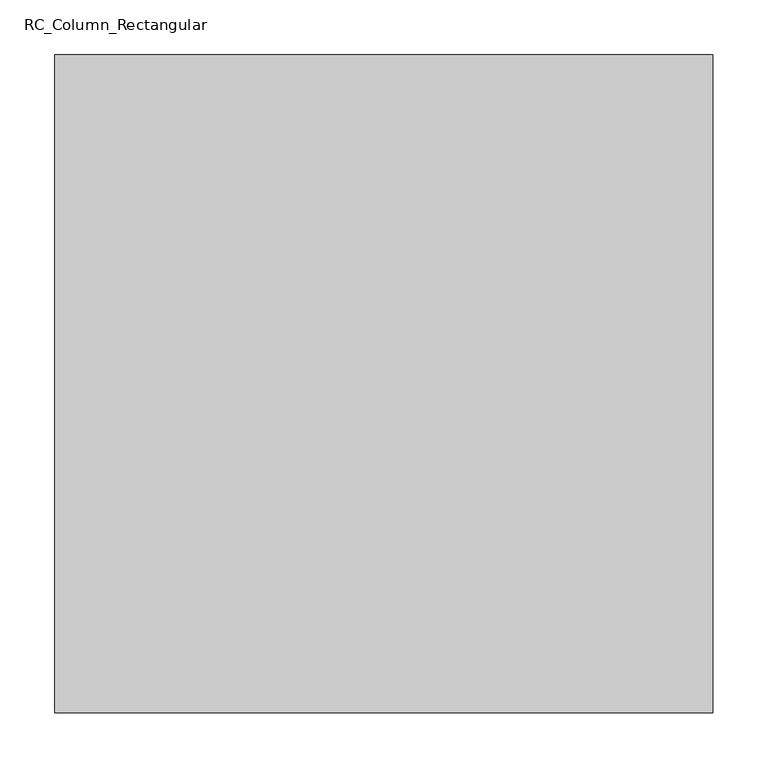
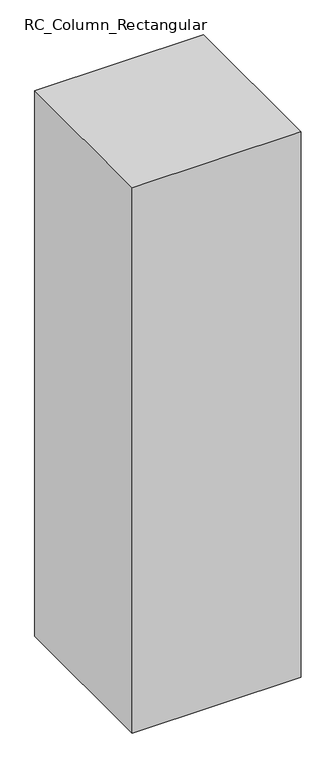
"""IFC4 building model written with IfcOpenShell, lengths in millimetres: column geometry, RC_Column_Rectangular : H_SC_AR_S15_UG PED_W600xL600_Bit_PD2."""

import ifcopenshell
import ifcopenshell.guid

model = None  # the IFC model being written
_history = None  # IfcOwnerHistory: only IFC2X3 demands one
_inside = {}  # id of a spatial element -> (the spatial element, [elements in it])
_under = {}  # id of a project, library or spatial element -> (it, [spatial elements below it])
_declared = {}  # id of a project -> (the project, [libraries it declares])
_typed = {}  # id of a type object -> (the type object, [elements of that type])
_made_of = {}  # id of a material, layer set ... -> (it, [elements and type objects made of it])


def new_model(schema):
    """Start an empty IFC model of exactly this schema.

    Asked for "IFC4X3", IfcOpenShell would pick the latest addendum, in which some entities
    have other attributes; the version numbers below select the first issue.
    IFC2X3 requires an IfcOwnerHistory on every rooted entity: one is made here for all.
    """
    global model, _history
    if schema == "IFC4X3":
        model = ifcopenshell.file(schema_version=(4, 3, 0, 0))
    else:
        model = ifcopenshell.file(schema=schema)
    _inside.clear()
    _under.clear()
    _declared.clear()
    _typed.clear()
    _made_of.clear()
    _history = None
    if model.schema == "IFC2X3":
        org = make("IfcOrganization", Name="unknown")
        user = make(
            "IfcPersonAndOrganization",
            ThePerson=make("IfcPerson", FamilyName="unknown"),
            TheOrganization=org,
        )
        app = make(
            "IfcApplication",
            ApplicationDeveloper=org,
            Version="unknown",
            ApplicationFullName="unknown",
            ApplicationIdentifier="unknown",
        )
        _history = make(
            "IfcOwnerHistory",
            OwningUser=user,
            OwningApplication=app,
            ChangeAction="ADDED",
            CreationDate=0,
        )
    return model


def make(cls, **values):
    """One entity of the class cls with the attributes given. An attribute that is None is left unset."""
    return model.create_entity(
        cls, **{name: value for name, value in values.items() if value is not None}
    )


def rooted(cls, **values):
    """An entity with a GlobalId (a new one), such as an element, a storey or a relation."""
    return make(cls, GlobalId=ifcopenshell.guid.new(), OwnerHistory=_history, **values)


def si_unit(unit_type, name, prefix=None):
    """IfcSIUnit, for example si_unit("LENGTHUNIT", "METRE", prefix="MILLI")."""
    return make("IfcSIUnit", UnitType=unit_type, Prefix=prefix, Name=name)


def assignment(units):
    """IfcUnitAssignment: the units of a project."""
    return None if units is None else make("IfcUnitAssignment", Units=units)


def point(xyz):
    """IfcCartesianPoint."""
    return None if xyz is None else make("IfcCartesianPoint", Coordinates=xyz)


def direction(xyz):
    """IfcDirection."""
    return None if xyz is None else make("IfcDirection", DirectionRatios=xyz)


def frame(location, z_axis=None, x_axis=None):
    """IfcAxis2Placement3D, a coordinate frame: its origin and axes. An axis left out is left unset."""
    return make(
        "IfcAxis2Placement3D",
        Location=point(location),
        Axis=direction(z_axis),
        RefDirection=direction(x_axis),
    )


def origin():
    """The frame at (0, 0, 0) with its axes left unset."""
    return frame((0.0, 0.0, 0.0))


def place(relative_to, where):
    """IfcLocalPlacement: puts the frame where relative to a parent placement (None: the world)."""
    return make(
        "IfcLocalPlacement", PlacementRelTo=relative_to, RelativePlacement=where
    )


def context(
    kind, dimensions, precision=None, world=None, true_north=None, identifier=None
):
    """IfcGeometricRepresentationContext, for example the 3D "Model" context."""
    return make(
        "IfcGeometricRepresentationContext",
        ContextIdentifier=identifier,
        ContextType=kind,
        CoordinateSpaceDimension=dimensions,
        Precision=precision,
        WorldCoordinateSystem=world,
        TrueNorth=true_north,
    )


def project(units=None, contexts=None):
    """IfcProject with its units and contexts."""
    return rooted(
        "IfcProject",
        Name="project",
        RepresentationContexts=contexts,
        UnitsInContext=assignment(units),
    )


def spatial(cls, under=None, at=None, **own):
    """A site, building, storey or space (cls), placed at a placement, below another one or the project."""
    s = rooted(cls, ObjectPlacement=at, **own)
    if under is not None:
        _under.setdefault(under.id(), (under, []))[1].append(s)
    return s


def polyline(points):
    """IfcPolyline through the points."""
    return make("IfcPolyline", Points=[point(p) for p in points])


def outline(outer, holes=None, kind="AREA"):
    """IfcArbitraryClosedProfileDef: a profile drawn as a closed curve; with holes, ...WithVoids."""
    if holes is None:
        return make("IfcArbitraryClosedProfileDef", ProfileType=kind, OuterCurve=outer)
    return make(
        "IfcArbitraryProfileDefWithVoids",
        ProfileType=kind,
        OuterCurve=outer,
        InnerCurves=holes,
    )


def extrude(swept, where, along, depth):
    """IfcExtrudedAreaSolid: the profile swept, set in the frame where, extruded along a direction by depth."""
    return make(
        "IfcExtrudedAreaSolid",
        SweptArea=swept,
        Position=where,
        ExtrudedDirection=direction(along),
        Depth=depth,
    )


def shape(context_of_items, identifier, shape_type, items):
    """IfcShapeRepresentation: the items that make up one representation, for example the "Body"."""
    return make(
        "IfcShapeRepresentation",
        ContextOfItems=context_of_items,
        RepresentationIdentifier=identifier,
        RepresentationType=shape_type,
        Items=items,
    )


def source(mapping_origin, context_of_items, identifier, shape_type, items):
    """IfcRepresentationMap: a shape defined once, which mapped items show again and again."""
    return make(
        "IfcRepresentationMap",
        MappingOrigin=mapping_origin,
        MappedRepresentation=shape(context_of_items, identifier, shape_type, items),
    )


def transform(
    local_origin,
    x_axis=None,
    y_axis=None,
    z_axis=None,
    scale=None,
    scale2=None,
    scale3=None,
    uniform=True,
):
    """IfcCartesianTransformationOperator3D, or its non-uniform kind. x_axis, y_axis, z_axis: its Axis1, 2, 3."""
    if uniform:
        return make(
            "IfcCartesianTransformationOperator3D",
            Axis1=direction(x_axis),
            Axis2=direction(y_axis),
            LocalOrigin=point(local_origin),
            Scale=scale,
            Axis3=direction(z_axis),
        )
    return make(
        "IfcCartesianTransformationOperator3DnonUniform",
        Axis1=direction(x_axis),
        Axis2=direction(y_axis),
        LocalOrigin=point(local_origin),
        Scale=scale,
        Axis3=direction(z_axis),
        Scale2=scale2,
        Scale3=scale3,
    )


def mapped(mapping_source, mapping_target):
    """IfcMappedItem: shows the shape of a source again, moved by a transform."""
    return make(
        "IfcMappedItem", MappingSource=mapping_source, MappingTarget=mapping_target
    )


def made_of(thing, what):
    """Note that an element or type object is made of a material, layer set ...; save() writes the relation."""
    if what is not None:
        _made_of.setdefault(what.id(), (what, []))[1].append(thing)
    return thing


def element(
    cls,
    number,
    at=None,
    inside=None,
    cuts=None,
    type_object=None,
    material=None,
    context=None,
    identifier="Body",
    shape_type=None,
    held_by="IfcProductDefinitionShape",
    body=None,
    shapes=None,
    **own,
):
    """One element of the class cls, such as IfcWall. Its Tag is "e" and its number.

    at: its placement. inside: the storey or other place that contains it. cuts: it is an
    opening in that element (IfcRelVoidsElement). A single representation is given by context,
    identifier, shape_type and body (its items); several are given by shapes. held_by: the class
    of the entity that holds the representations. save() writes the other relations.
    """
    e = rooted(cls, Tag="e%d" % number, ObjectPlacement=at, **own)
    if body is not None:
        shapes = [shape(context, identifier, shape_type, body)]
    if shapes is not None:
        e.Representation = make(held_by, Representations=shapes)
    if inside is not None:
        _inside.setdefault(inside.id(), (inside, []))[1].append(e)
    if cuts is not None:
        rooted(
            "IfcRelVoidsElement", RelatingBuildingElement=cuts, RelatedOpeningElement=e
        )
    if type_object is not None:
        _typed.setdefault(type_object.id(), (type_object, []))[1].append(e)
    return made_of(e, material)


def aggregate(whole, parts):
    """IfcRelAggregates: a whole, such as a stair, and the parts it consists of."""
    return rooted("IfcRelAggregates", RelatingObject=whole, RelatedObjects=parts)


def save(model, path):
    """Write the relations noted so far, then the file.

    IfcRelAggregates (storeys below a building ...), IfcRelContainedInSpatialStructure (elements
    in a storey), IfcRelDefinesByType, IfcRelAssociatesMaterial and IfcRelDeclares: one each for
    every whole, place, type object, material and project.
    """
    for whole, parts in _under.values():
        aggregate(whole, parts)
    for where, things in _inside.values():
        rooted(
            "IfcRelContainedInSpatialStructure",
            RelatedElements=things,
            RelatingStructure=where,
        )
    for kind, things in _typed.values():
        rooted("IfcRelDefinesByType", RelatedObjects=things, RelatingType=kind)
    for what, things in _made_of.values():
        rooted("IfcRelAssociatesMaterial", RelatedObjects=things, RelatingMaterial=what)
    for by, libraries in _declared.values():
        rooted("IfcRelDeclares", RelatingContext=by, RelatedDefinitions=libraries)
    model.write(path)


def rc_column_rectangular_fa199b6f(model_context):
    return source(origin(), model_context, "Body", "SweptSolid", [
        extrude(outline(polyline([(300.0, 300.0), (300.0, -300.0), (-300.0, -300.0), (-300.0, 300.0), (300.0, 300.0)])), frame((0.0, 0.0, -9380.1756499), z_axis=(0.0, 0.0, 1.0), x_axis=(1.0, 0.0, 0.0)), (0.0, 0.0, 1.0), 2050.0),
    ])


if __name__ == "__main__":
    model = new_model("IFC4")
    model_context = context("Model", 3, world=origin())
    ifc_project = project(units=[si_unit("LENGTHUNIT", "METRE", prefix="MILLI")], contexts=[model_context])
    site = spatial("IfcSite", under=ifc_project)
    building = spatial("IfcBuilding", under=site)
    placement = place(None, origin())
    rc_column_rectangular_shape = rc_column_rectangular_fa199b6f(model_context)
    element("IfcColumn", 1, ObjectType="RC_Column_Rectangular : H_SC_AR_S15_UG PED_W600xL600_Bit_PD2", at=placement, inside=building, context=model_context, shape_type="MappedRepresentation", body=[
        mapped(rc_column_rectangular_shape, transform((0.0, 0.0, 0.0), x_axis=(1.0, 0.0, 0.0), y_axis=(0.0, 1.0, 0.0), z_axis=(0.0, 0.0, 1.0))),
    ])
    save(model, "model.ifc")

# Revit data of these elements
# Type "RC_Column_Rectangular : H_SC_AR_S15_UG PED_W600xL600_Bit_PD2"
#   Type Mark = "PD2"
#   Width = 600 mm
#   Length = 600 mm
#   hec_material3 [instance default] = none
#   hec_material2 [instance default] = none
#   hec_material1 [instance default] = none
#   Structural Material [instance default] = none
#   Description = (empty or 0)
